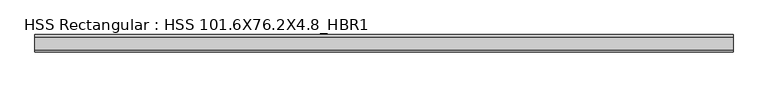
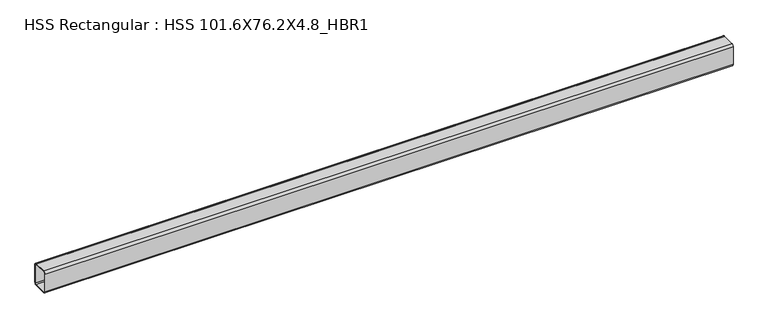
"""IFC4 building model written with IfcOpenShell, lengths in millimetres: beam geometry, HSS Rectangular : HSS 101.6X76.2X4.8_HBR1."""

from ifc_helpers import new_model, si_unit, point, frame, frame_2d, origin, place, context, project, spatial, polyline, circle_curve, trimmed, segment, composite_curve, outline, extrude, source, transform, mapped, element, save


def hss_rectangular_hss_101_6x76_2x4_8_hbr1_1636cf47(model_context):
    return source(origin(), model_context, "Body", "SweptSolid", [
        extrude(outline(composite_curve([segment(polyline([(38.1, 41.275), (38.1, -41.275)]), True, "CONTINUOUS"), segment(trimmed(circle_curve(frame_2d((28.575, -41.275)), 9.525), [point((38.1, -41.275))], [point((28.575, -50.8))], False, "CARTESIAN"), True, "CONTINUOUS"), segment(polyline([(28.575, -50.8), (-28.575, -50.8)]), True, "CONTINUOUS"), segment(trimmed(circle_curve(frame_2d((-28.575, -41.275)), 9.525), [point((-28.575, -50.8))], [point((-38.1, -41.275))], False, "CARTESIAN"), True, "CONTINUOUS"), segment(polyline([(-38.1, -41.275), (-38.1, 41.275)]), True, "CONTINUOUS"), segment(trimmed(circle_curve(frame_2d((-28.575, 41.275)), 9.525), [point((-38.1, 41.275))], [point((-28.575, 50.8))], False, "CARTESIAN"), True, "CONTINUOUS"), segment(polyline([(-28.575, 50.8), (28.575, 50.8)]), True, "CONTINUOUS"), segment(trimmed(circle_curve(frame_2d((28.575, 41.275)), 9.525), [point((28.575, 50.8))], [point((38.1, 41.275))], False, "CARTESIAN"), True, "CONTINUOUS")], self_intersect=False), holes=[composite_curve([segment(trimmed(circle_curve(frame_2d((-28.575, 41.275)), 4.7625), [point((-28.575, 46.0375))], [point((-33.3375, 41.275))], True, "CARTESIAN"), True, "CONTINUOUS"), segment(polyline([(-33.3375, 41.275), (-33.3375, -41.275)]), True, "CONTINUOUS"), segment(trimmed(circle_curve(frame_2d((-28.575, -41.275)), 4.7625), [point((-33.3375, -41.275))], [point((-28.575, -46.0375))], True, "CARTESIAN"), True, "CONTINUOUS"), segment(polyline([(-28.575, -46.0375), (28.575, -46.0375)]), True, "CONTINUOUS"), segment(trimmed(circle_curve(frame_2d((28.575, -41.275)), 4.7625), [point((28.575, -46.0375))], [point((33.3375, -41.275))], True, "CARTESIAN"), True, "CONTINUOUS"), segment(polyline([(33.3375, -41.275), (33.3375, 41.275)]), True, "CONTINUOUS"), segment(trimmed(circle_curve(frame_2d((28.575, 41.275)), 4.7625), [point((33.3375, 41.275))], [point((28.575, 46.0375))], True, "CARTESIAN"), True, "CONTINUOUS"), segment(polyline([(28.575, 46.0375), (-28.575, 46.0375)]), True, "CONTINUOUS")], self_intersect=False)]), frame((-1575.1664516, 0.0, 0.0), z_axis=(1.0, 0.0, 0.0), x_axis=(0.0, 1.0, 0.0)), (0.0, 0.0, 1.0), 3053.3977307),
    ])


if __name__ == "__main__":
    model = new_model("IFC4")
    model_context = context("Model", 3, world=origin())
    ifc_project = project(units=[si_unit("LENGTHUNIT", "METRE", prefix="MILLI")], contexts=[model_context])
    site = spatial("IfcSite", under=ifc_project)
    building = spatial("IfcBuilding", under=site)
    placement = place(None, origin())
    hss_rectangular_hss_101_6x76_2x4_8_hbr1_shape = hss_rectangular_hss_101_6x76_2x4_8_hbr1_1636cf47(model_context)
    element("IfcBeam", 1, ObjectType="HSS Rectangular : HSS 101.6X76.2X4.8_HBR1", at=placement, inside=building, context=model_context, shape_type="MappedRepresentation", body=[
        mapped(hss_rectangular_hss_101_6x76_2x4_8_hbr1_shape, transform((0.0, 0.0, 0.0), x_axis=(1.0, 0.0, 0.0), y_axis=(0.0, 1.0, 0.0), z_axis=(0.0, 0.0, 1.0))),
    ])
    save(model, "model.ifc")

# Revit data of these elements
# Type "HSS Rectangular : HSS 101.6X76.2X4.8_HBR1"
#   Section Name Key = "HSS 4X3X3/16"
#   Assembly Code = "B10"
#   Width = 7.62 cm
#   Wall Nominal Thickness = 0.4763 cm
#   Wall Design Thickness = 0.442 cm
#   Torsional Moment of Inertia = 260.561 cm⁴
#   Torsional Modulus = 61.2876 cm³
#   Section Area = 14.4516 cm²
#   Plastic Modulus weak axis = 40.3122 cm³
#   Plastic Modulus strong axis = 49.1612 cm³
#   Perimeter = 0.881482 m²/m
#   Outer Fillet = 0.9525 cm
#   Nominal Weight = 12.1285 kgf/m
#   Moment of Inertia weak axis = 131.529 cm⁴
#   Moment of Inertia strong axis = 205.202 cm⁴
#   Inner Fillet = 0.4763 cm
#   Height = 10.16 cm
#   Elastic Modulus weak axis = 34.4128 cm³
#   Elastic Modulus strong axis = 40.476 cm³
#   Centroid Vertical = 5.08 cm
#   Centroid Horizontal = 3.81 cm
#   Length [instance default] = 1524 mm
#   Structural Material [instance default] = Steel ASTM A500, Grade B, Rectangular and Square
#   Principal Axes Angle = 0
# Element 1 (IfcBeam, "HSS Rectangular : HSS 101.6X76.2X4.8_HBR1")
#   Structural Material = Steel ASTM A992
#   Materials on its faces: "Steel ASTM A992"
# Materials
#   "Steel ASTM A500, Grade B, Rectangular and Square": class "Metal", colour RGB 199 199 199, transparency 0, Description = "Carbon steel", Cost = 0
#   "Steel ASTM A992": class "Metal", colour RGB 199 199 199, transparency 0, Description = "Structural steel 50ksi", Cost = 0
